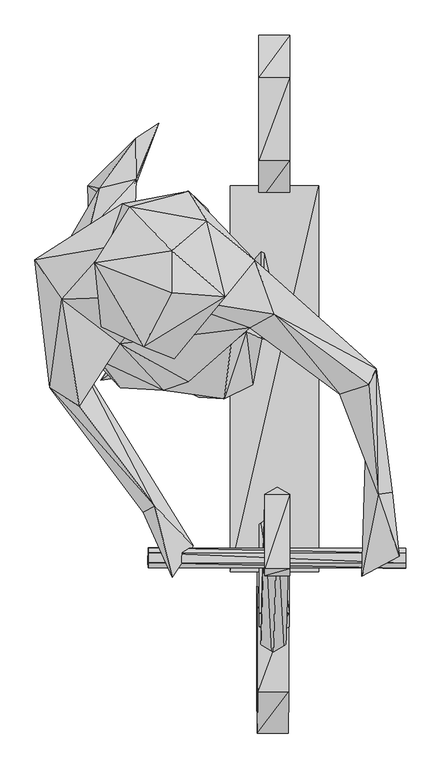
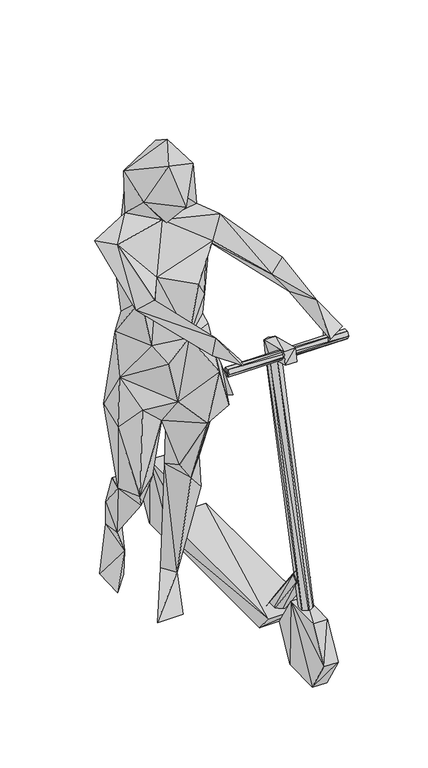
"""IFC4 building model written with IfcOpenShell, lengths in millimetres: geographic element geometry, Enscape AssetDefinition - Anita 001 Scooter : Enscape AssetDefinition - Anita 001 Scooter."""

from ifc_helpers import new_model, si_unit, origin, place, context, project, spatial, faceted_brep, source, transform, mapped, element, save


def geographic_element_0ec8fd72(model_context):
    return source(origin(), model_context, "Body", "Brep", [
        faceted_brep([(25.2, 461.9559944, -0.35), (-25.2, 530.36201, 118.1320027), (25.2, 530.36201, 118.1320027), (-25.2, 461.9559944, -0.35), (-25.2, 461.9559944, 236.6160005), (25.2, 325.1439929, -0.35), (25.2, 461.9559944, 236.6160005), (-25.2, 325.1439929, -0.35), (-25.2, 325.1430094, 236.6160005), (-25.2, 256.7380071, 118.1320027), (25.2, 325.1430094, 236.6160005), (25.2, 256.7380071, 118.1320027)], [[[0, 1, 2]], [[3, 1, 0]], [[1, 4, 2]], [[3, 4, 1]], [[2, 5, 0]], [[6, 5, 2]], [[2, 4, 6]], [[5, 3, 0]], [[7, 3, 5]], [[7, 4, 3]], [[4, 8, 6]], [[9, 4, 7]], [[4, 9, 8]], [[10, 5, 6]], [[6, 8, 10]], [[11, 7, 5]], [[5, 10, 11]], [[9, 7, 11]], [[10, 9, 11]], [[8, 9, 10]]]),
        faceted_brep([(72.0719993, 285.1270139, 84.4769999), (-72.0719993, -290.6019986, 84.4769999), (-72.0719993, 285.1270139, 84.4769999), (72.0719993, -290.6019986, 84.4769999), (-72.0719993, -344.4449902, 147.7800012), (72.0719993, -344.4449902, 147.7800012), (-72.0719993, 285.1270139, 147.7800012), (72.0719993, 285.1270139, 147.7800012)], [[[0, 1, 2]], [[3, 1, 0]], [[4, 2, 1]], [[5, 1, 3]], [[4, 1, 5]], [[6, 2, 4]], [[6, 0, 2]], [[7, 3, 0]], [[7, 0, 6]], [[5, 3, 7]], [[7, 4, 5]], [[6, 4, 7]]]),
        faceted_brep([(-2.7979999, -463.2300138, 94.8520005), (-23.0810009, -497.2440004, 103.6520004), (-23.0810009, -474.5410085, 97.8889987), (4.619, -217.8930044, 1043.6480045), (-15.6640001, -229.203999, 1046.6840267), (17.4860004, -474.6200144, 97.5790024), (24.9029994, -229.283005, 1046.3739634), (4.9820002, -206.5369934, 1088.381052), (25.2659991, -217.926994, 1091.1079645), (-15.6629998, -251.9060075, 1052.4469614), (-15.3010003, -217.8480029, 1091.416955), (-15.2989998, -339.933008, 1122.4089861), (24.9029994, -251.9840002, 1052.1370173), (24.9049999, -351.3660133, 1077.3650408), (25.2679996, -340.0099874, 1122.0990419), (4.6199998, -263.2960081, 1055.1730394), (17.4870007, -497.3219931, 103.3419967), (-15.6619996, -351.2879908, 1077.6749849), (-2.7960001, -508.6330175, 106.3790023)], [[[0, 1, 2]], [[3, 2, 4]], [[0, 2, 3]], [[2, 1, 4]], [[5, 1, 0]], [[6, 0, 3]], [[5, 0, 6]], [[3, 4, 7]], [[8, 3, 7]], [[6, 3, 8]], [[4, 9, 10]], [[7, 4, 10]], [[4, 1, 9]], [[10, 8, 7]], [[10, 9, 11]], [[11, 8, 10]], [[12, 6, 8]], [[13, 8, 14]], [[12, 8, 13]], [[8, 11, 14]], [[12, 5, 6]], [[15, 16, 12]], [[16, 5, 12]], [[12, 17, 15]], [[17, 12, 13]], [[13, 14, 17]], [[17, 14, 11]], [[11, 9, 17]], [[15, 17, 9]], [[18, 16, 15]], [[9, 18, 15]], [[1, 18, 9]], [[1, 16, 18]], [[16, 1, 5]]]),
        faceted_brep([(21.7930004, -400.7610083, -0.927), (-27.5669992, -333.5489929, 118.6719984), (22.8310004, -333.6459994, 118.2880029), (-28.6069997, -400.6640017, -0.543), (-26.8019997, -403.2379985, 236.402005), (21.5179995, -537.5639796, -2.412), (23.5959999, -403.335005, 236.0170037), (-28.8800001, -537.4670029, -2.0270001), (-27.0760003, -540.0419831, 234.9179983), (-28.1150006, -607.156992, 115.7030016), (23.3219992, -540.1390195, 234.532997), (22.2830009, -607.2540283, 115.3180003)], [[[0, 1, 2]], [[3, 1, 0]], [[1, 4, 2]], [[3, 4, 1]], [[2, 5, 0]], [[6, 5, 2]], [[2, 4, 6]], [[5, 3, 0]], [[7, 3, 5]], [[7, 4, 3]], [[4, 8, 6]], [[9, 4, 7]], [[4, 9, 8]], [[10, 5, 6]], [[6, 8, 10]], [[11, 7, 5]], [[5, 10, 11]], [[9, 7, 11]], [[10, 9, 11]], [[8, 9, 10]]]),
        faceted_brep([(-24.6440005, -246.0269928, 120.9079996), (0.0, -400.2330005, 349.5759964), (0.0, -234.6570045, 129.4610053), (-24.6440005, -411.6039872, 341.0229981), (24.6440005, -411.6039872, 341.0229981), (-24.6440005, -268.768996, 103.8009971), (24.6440005, -246.0269928, 120.9079996), (-24.6440005, -434.3450069, 323.9159882), (24.6440005, -434.3450069, 323.9159882), (0.0, -445.7159936, 315.3620064), (24.6440005, -268.768996, 103.8009971), (0.0, -280.1400125, 95.2479988)], [[[0, 1, 2]], [[3, 1, 0]], [[1, 4, 2]], [[3, 4, 1]], [[2, 5, 0]], [[6, 5, 2]], [[2, 4, 6]], [[5, 3, 0]], [[7, 3, 5]], [[7, 4, 3]], [[4, 8, 6]], [[9, 4, 7]], [[4, 9, 8]], [[10, 5, 6]], [[6, 8, 10]], [[11, 7, 5]], [[5, 10, 11]], [[9, 7, 11]], [[10, 9, 11]], [[8, 9, 10]]]),
        faceted_brep([(213.8829976, -330.3439915, 1083.2979679), (-205.8600038, -337.8889859, 1100.6120443), (-205.9510052, -329.5370042, 1086.5030289), (213.9749974, -338.696003, 1097.4069834), (-205.734998, -329.847008, 1114.8990393), (213.9160037, -313.9489889, 1083.4759474), (214.0409946, -305.9059978, 1097.7619886), (214.1329944, -314.2580092, 1111.8710041), (214.0990049, -330.6519985, 1111.6939783), (-205.7020068, -313.4520054, 1115.0770187), (-205.7940066, -305.1010072, 1100.9680033), (-205.9179991, -313.1439984, 1086.6810083)], [[[0, 1, 2]], [[3, 1, 0]], [[3, 4, 1]], [[4, 2, 1]], [[0, 2, 5]], [[5, 3, 0]], [[6, 3, 5]], [[7, 3, 6]], [[3, 7, 8]], [[8, 4, 3]], [[8, 9, 4]], [[9, 2, 4]], [[7, 9, 8]], [[7, 10, 9]], [[6, 10, 7]], [[6, 11, 10]], [[5, 11, 6]], [[5, 2, 11]], [[2, 10, 11]], [[10, 2, 9]]]),
        faceted_brep([(-213.9640003, -247.2500056, 1119.67206), (-132.4249953, -301.9819856, 1094.6700573), (-166.7519957, -353.4809947, 1130.8859587), (-320.2759922, 3.7469999, 1210.9600306), (-194.8660016, -238.1139994, 1173.1319427), (-366.0829961, -44.8039994, 1219.1009521), (-317.8960085, -74.4270012, 1259.08494), (-311.2899959, 184.3879968, 1250.5949736), (-390.2510107, 164.3390059, 1360.9369993), (-346.8460143, 99.2640033, 1368.9620495), (-251.7989874, 26.912, 1259.8990202), (-188.2690042, 104.8870012, 1402.9179811), (-271.559, 184.4529957, 1410.4369879), (-247.6149946, 254.9239993, 1311.259985), (-293.8260138, 172.4330038, 1059.7980022), (-192.7399933, 200.7859945, 1136.4400387), (-139.3180043, 275.5919993, 1227.8740406), (-216.8669999, 257.0860088, 1120.3039885), (-235.4529947, 250.7100105, 1454.5109272), (-200.4639953, 179.6350032, 1021.1520195), (-332.9870105, 139.9549991, 1018.9529657), (-268.4850097, 201.0840029, 920.0479984), (-91.9670016, 107.431002, 1019.3719864), (-363.0929887, 158.1220031, 748.3459711), (-357.5929999, 70.4360008, 896.8709707), (-285.1960063, -0.036, 1032.9289436), (-251.0409951, -44.5890017, 977.8299928), (-181.0770035, -48.5140011, 1055.4950237), (-140.4539943, -34.8859988, 1231.752038), (-40.1719995, 53.413, 1305.3660393), (-62.2389987, 56.0920015, 1229.8020124), (-55.2040003, 73.6849979, 1102.5429964), (0.012, 74.8369992, 1378.2320023), (106.7159995, -55.594001, 1194.3830252), (-24.2340006, 100.7049978, 1267.6390409), (-77.1609992, 173.6250073, 1217.0419693), (-31.9660008, 162.8610045, 1374.5589256), (150.4860073, -85.0140005, 1134.0579987), (165.7049954, -13.8020003, 1182.7830076), (153.4589976, -39.5129994, 1232.5400114), (169.0189987, -218.3759958, 1176.0259867), (191.967994, -215.3050005, 1133.5690022), (142.2629952, -351.4750004, 1120.4919815), (203.7899941, -319.1890121, 1126.6729832), (-80.0660029, 103.6449969, 1577.0769119), (-126.0229945, 94.0579996, 1485.6200218), (-110.0779995, 227.7940065, 1411.3279581), (-108.893998, 246.6299981, 1148.211956), (-167.3820019, 178.2789975, 1647.3129988), (-292.6470041, 158.9590013, 1590.1670456), (-167.493999, 110.4829982, 1692.8119659), (-282.3120058, 54.8320003, 1532.8429937), (-212.8880024, 22.0759995, 1660.9669924), (-193.1529939, 66.3319975, 1418.4559584), (-163.0659997, 2.4319999, 1503.4769773), (-73.7579986, 53.9949983, 1045.7489491), (-70.2370033, 27.9869996, 1024.3799686), (-52.2670001, 141.6579932, 825.3930211), (-45.8020009, 46.7020012, 924.9550104), (-203.204006, -18.2440002, 806.0960174), (-81.3490003, -62.3989999, 901.2190104), (-35.1389982, -39.6439992, 749.5359778), (-20.3900002, 35.441, 851.0550261), (-123.1739968, -60.2370016, 723.4899998), (-19.3530004, 50.8319996, 726.4900208), (17.6660009, 28.4150001, 727.2549868), (-16.1889996, 174.5740026, 737.6019955), (-21.2830007, 177.3039997, 879.0820241), (-76.549001, 71.3049993, 506.7679882), (-122.4370003, 40.0170013, 460.4890049), (-97.7649987, 138.7809962, 529.6490192), (-101.4140025, 124.7399971, 722.8429914), (-51.4580011, 102.3410037, 365.437001), (-124.6159971, 156.7209959, 377.6949942), (-169.6310043, 120.6170022, 480.9730053), (-182.7590019, 88.1600007, 686.5879893), (-167.4720049, 197.0899999, 851.3550162), (-213.8399929, 150.1570046, 692.1049953), (-276.4799893, 197.8379935, 720.5920219), (-219.0839946, 54.4140004, 698.0389953), (-170.8090007, 26.0979999, 533.3009958), (-269.8740065, 117.794998, 495.7489967), (-347.694993, 96.3689983, 465.5250013), (-233.4509939, 87.0610029, 473.0139971), (-301.6459942, 211.9120061, 417.9230034), (-224.9370068, 295.2359915, 215.2830064), (-323.1930137, 2.8270001, 481.2920094), (-242.7780032, 138.6139989, 339.1329944), (-347.8960097, 173.0179936, 368.1229949), (-285.6880128, 280.8740139, 200.5690038), (-304.1040003, 284.5650017, 16.9580001), (-240.7190055, 242.1659976, 107.2719991), (-277.7810097, 224.3999988, 200.1609951), (-225.5309969, 362.5290096, 170.5480069), (-372.7299869, 54.0219992, 726.7439961), (-308.4999919, 14.7360004, 791.4810181), (-163.3079946, 55.3839989, 113.3510023), (-195.2069998, 100.5420014, 114.3470034), (-220.540002, 63.0030036, 0.906), (-283.066988, -32.5150006, 20.3380007), (-140.5729949, 166.6200012, 75.6810009), (-128.3939928, 132.190004, 161.6649926), (-124.3039966, 149.4449973, -4.2340001), (-183.7259978, -17.2380004, 8.4819999), (-238.6270016, 252.5019944, 11.9160004), (-300.7900119, 181.1890006, 8.5009998), (-188.737005, 386.465013, 67.2879964), (142.4410045, -312.5990033, 1074.1920471)], [[[0, 1, 2]], [[3, 1, 0]], [[4, 1, 3]], [[1, 4, 2]], [[4, 0, 2]], [[5, 3, 0]], [[5, 0, 4]], [[4, 6, 5]], [[3, 6, 4]], [[7, 3, 5]], [[8, 7, 5]], [[9, 5, 6]], [[5, 9, 8]], [[10, 9, 6]], [[3, 10, 6]], [[11, 12, 9]], [[11, 9, 10]], [[12, 8, 9]], [[12, 13, 8]], [[8, 13, 7]], [[14, 3, 7]], [[13, 14, 7]], [[13, 15, 14]], [[13, 16, 17]], [[18, 13, 12]], [[13, 17, 15]], [[13, 18, 16]], [[14, 15, 19]], [[3, 14, 20]], [[20, 14, 19]], [[19, 21, 20]], [[21, 19, 22]], [[15, 22, 19]], [[23, 24, 20]], [[20, 24, 25]], [[21, 23, 20]], [[20, 25, 3]], [[25, 10, 3]], [[25, 24, 26]], [[25, 26, 27]], [[10, 25, 27]], [[28, 10, 27]], [[11, 10, 29]], [[29, 10, 28]], [[28, 30, 29]], [[30, 28, 31]], [[31, 28, 27]], [[32, 11, 29]], [[29, 33, 32]], [[30, 34, 29]], [[34, 33, 29]], [[34, 30, 31]], [[35, 36, 34]], [[34, 37, 33]], [[35, 34, 31]], [[34, 38, 37]], [[34, 36, 38]], [[39, 33, 40]], [[32, 33, 39]], [[40, 33, 37]], [[38, 41, 37]], [[40, 37, 42]], [[42, 37, 41]], [[40, 42, 43]], [[39, 40, 38]], [[41, 38, 40]], [[41, 40, 43]], [[38, 36, 32]], [[38, 32, 39]], [[44, 45, 36]], [[36, 35, 16]], [[36, 45, 11]], [[36, 11, 32]], [[16, 46, 36]], [[36, 46, 44]], [[18, 46, 16]], [[16, 47, 17]], [[16, 35, 47]], [[46, 18, 48]], [[46, 48, 44]], [[18, 12, 49]], [[49, 48, 18]], [[49, 50, 48]], [[48, 50, 44]], [[12, 51, 49]], [[50, 49, 52]], [[52, 49, 51]], [[11, 51, 12]], [[11, 53, 51]], [[51, 53, 54]], [[52, 51, 54]], [[52, 54, 44]], [[52, 44, 50]], [[54, 45, 44]], [[45, 54, 53]], [[53, 11, 45]], [[17, 47, 15]], [[47, 35, 15]], [[35, 31, 15]], [[15, 31, 22]], [[31, 27, 55]], [[22, 31, 55]], [[55, 56, 22]], [[57, 22, 58]], [[58, 22, 56]], [[21, 22, 57]], [[56, 55, 27]], [[26, 59, 27]], [[27, 59, 60]], [[56, 27, 60]], [[56, 60, 58]], [[58, 60, 61]], [[58, 61, 62]], [[62, 57, 58]], [[60, 59, 63]], [[61, 60, 63]], [[63, 64, 61]], [[64, 62, 61]], [[62, 64, 65]], [[66, 62, 65]], [[62, 67, 57]], [[66, 67, 62]], [[66, 65, 64]], [[66, 64, 57]], [[67, 66, 57]], [[68, 64, 69]], [[70, 64, 68]], [[57, 64, 71]], [[69, 64, 63]], [[70, 71, 64]], [[68, 69, 72]], [[70, 68, 72]], [[70, 72, 73]], [[70, 74, 75]], [[75, 71, 70]], [[74, 70, 73]], [[75, 76, 71]], [[76, 57, 71]], [[21, 57, 76]], [[76, 75, 77]], [[78, 76, 77]], [[78, 21, 76]], [[79, 75, 80]], [[77, 75, 79]], [[75, 74, 80]], [[81, 77, 79]], [[77, 81, 78]], [[23, 78, 82]], [[82, 78, 81]], [[21, 78, 23]], [[81, 83, 84]], [[82, 81, 84]], [[81, 79, 83]], [[84, 83, 85]], [[83, 86, 87]], [[86, 83, 79]], [[85, 83, 87]], [[88, 84, 89]], [[84, 88, 82]], [[84, 85, 89]], [[89, 90, 91]], [[89, 92, 88]], [[89, 91, 92]], [[93, 90, 89]], [[85, 93, 89]], [[88, 92, 82]], [[92, 87, 82]], [[92, 85, 87]], [[91, 85, 92]], [[86, 82, 87]], [[82, 86, 94]], [[23, 82, 94]], [[86, 95, 94]], [[24, 94, 95]], [[24, 23, 94]], [[79, 95, 86]], [[24, 95, 59]], [[95, 79, 59]], [[26, 24, 59]], [[59, 79, 63]], [[79, 80, 63]], [[63, 80, 69]], [[74, 69, 80]], [[74, 96, 69]], [[96, 72, 69]], [[74, 97, 96]], [[74, 73, 97]], [[98, 99, 97]], [[100, 98, 97]], [[96, 97, 99]], [[97, 101, 100]], [[97, 73, 101]], [[73, 72, 101]], [[101, 72, 96]], [[100, 101, 96]], [[100, 102, 98]], [[100, 96, 102]], [[102, 103, 98]], [[98, 103, 99]], [[103, 96, 99]], [[102, 96, 103]], [[85, 91, 104]], [[91, 90, 105]], [[104, 91, 105]], [[90, 104, 105]], [[90, 106, 104]], [[104, 106, 85]], [[93, 85, 106]], [[93, 106, 90]], [[41, 43, 107]], [[42, 41, 107]], [[107, 43, 42]]]),
    ])


if __name__ == "__main__":
    model = new_model("IFC4")
    model_context = context("Model", 3, world=origin())
    ifc_project = project(units=[si_unit("LENGTHUNIT", "METRE", prefix="MILLI")], contexts=[model_context])
    site = spatial("IfcSite", under=ifc_project)
    building = spatial("IfcBuilding", under=site)
    placement = place(None, origin())
    geographic_element_shape = geographic_element_0ec8fd72(model_context)
    element("IfcGeographicElement", 1, ObjectType="Enscape AssetDefinition - Anita 001 Scooter : Enscape AssetDefinition - Anita 001 Scooter", at=placement, inside=building, context=model_context, shape_type="MappedRepresentation", body=[
        mapped(geographic_element_shape, transform((0.0, 0.0, 0.0), x_axis=(1.0, 0.0, 0.0), y_axis=(0.0, 1.0, 0.0), z_axis=(0.0, 0.0, 1.0))),
    ])
    save(model, "model.ifc")

# Revit data of these elements
# Type "Enscape AssetDefinition - Anita 001 Scooter : Enscape AssetDefinition - Anita 001 Scooter"
#   EnscapeAssetSource = "REMOTE"
#   EnscapeAssetId = "b95b1418-837d-4387-8a94-8f592f43e25a"
#   Height = 1692.812 mm
#   EnscapeNativeAssetHeight = 1692.812 mm
#   Default Elevation = 0
